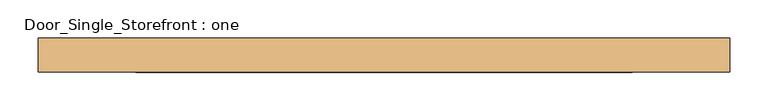
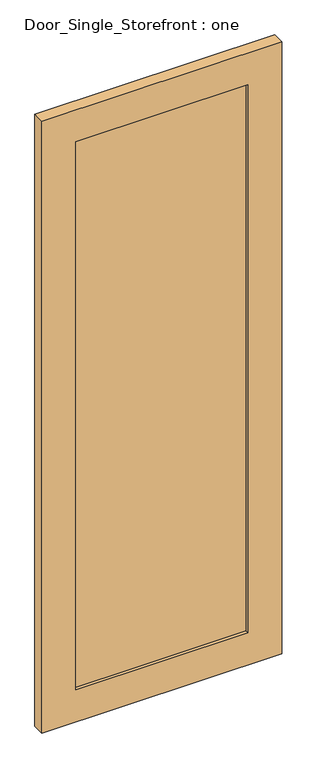
"""IFC4 building model written with IfcOpenShell, lengths in millimetres: door geometry, Door_Single_Storefront : one."""

from ifc_helpers import new_model, si_unit, frame, origin, place, context, project, spatial, polyline, outline, extrude, source, transform, mapped, element, save


def door_single_storefront_one_eb725c03(model_context):
    return source(origin(), model_context, "Body", "SweptSolid", [
        extrude(outline(polyline([(323.85, -6.35), (-323.85, -6.35), (-323.85, 12.7), (323.85, 12.7), (323.85, -6.35)])), frame((0.0, 0.0, 127.0), z_axis=(0.0, 0.0, 1.0), x_axis=(1.0, 0.0, 0.0)), (0.0, 0.0, 1.0), 2178.05),
        extrude(outline(polyline([(2432.05, -450.85), (0.0, -450.85), (0.0, 450.85), (2432.05, 450.85), (2432.05, -450.85)]), holes=[polyline([(127.0, 323.85), (127.0, -323.85), (2305.05, -323.85), (2305.05, 323.85), (127.0, 323.85)])]), frame((0.0, -19.05, 0.0), z_axis=(0.0, 1.0, 0.0), x_axis=(0.0, 0.0, 1.0)), (0.0, 0.0, 1.0), 44.45),
    ])


if __name__ == "__main__":
    model = new_model("IFC4")
    model_context = context("Model", 3, world=origin())
    ifc_project = project(units=[si_unit("LENGTHUNIT", "METRE", prefix="MILLI")], contexts=[model_context])
    site = spatial("IfcSite", under=ifc_project)
    building = spatial("IfcBuilding", under=site)
    placement = place(None, origin())
    door_single_storefront_one_shape = door_single_storefront_one_eb725c03(model_context)
    element("IfcDoor", 1, ObjectType="Door_Single_Storefront : one", at=placement, inside=building, context=model_context, shape_type="MappedRepresentation", body=[
        mapped(door_single_storefront_one_shape, transform((0.0, 0.0, 0.0), x_axis=(1.0, 0.0, 0.0), y_axis=(0.0, 1.0, 0.0), z_axis=(0.0, 0.0, 1.0))),
    ])
    save(model, "model.ifc")

# Revit data of these elements
# Type "Door_Single_Storefront : one"
#   Type Mark = "27"
#   Analytic Construction = "<None>"
#   Stile_Width = 0' - 5"
#   Door_Thickness = 0' - 1 3/4"
#   Door_Offset = 0' - 1"
#   Glass_Material = SAFETY GLAZING
#   Frame_Material = INTERIOR GRADE ALUMINUM STOREFRONT W/ SAFETY GLAZING
#   Function = (empty or 0)
# Element 1 (IfcDoor, "Door_Single_Storefront : one")
#   Materials on its faces: "INTERIOR GRADE ALUMINUM STOREFRONT W/ SAFETY GLAZING", "SAFETY GLAZING"
# Materials
#   "SAFETY GLAZING": class "Glass", colour RGB 142 168 196, transparency 0.75, Description = "Soda Lime Glass", Cost = 0
#   "INTERIOR GRADE ALUMINUM STOREFRONT W/ SAFETY GLAZING": class "Metal", colour RGB 226 226 226, transparency 0, Description = "Aluminum 6061", Cost = 0
